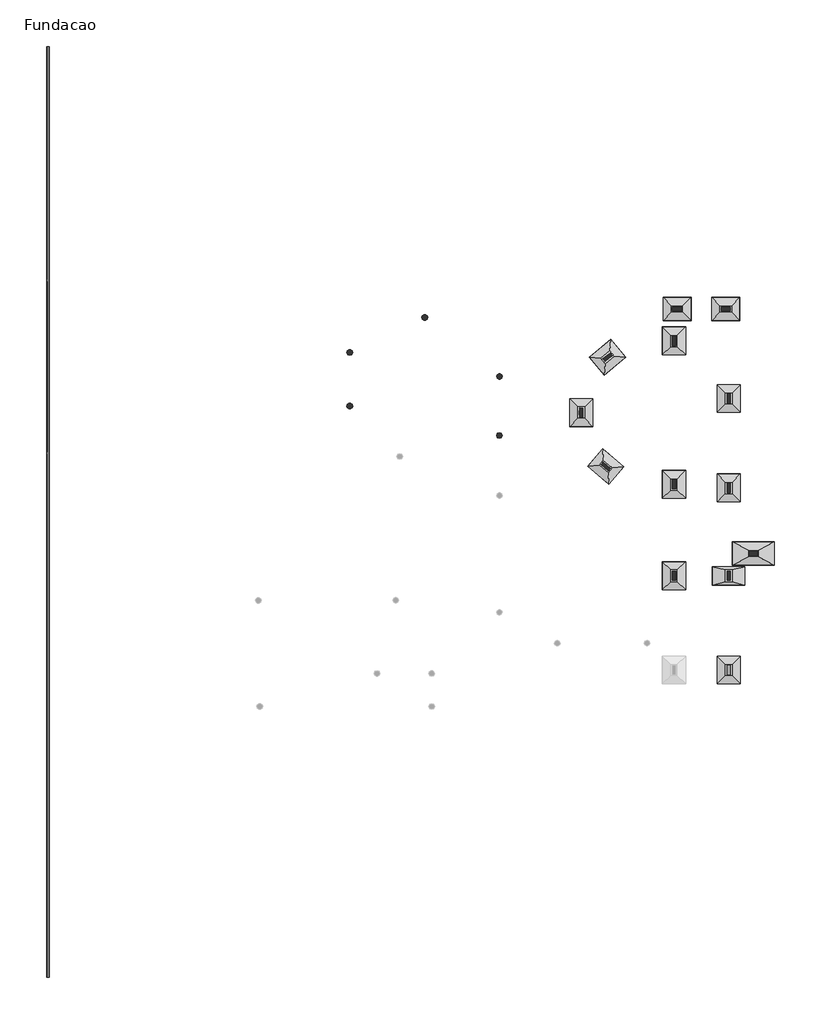
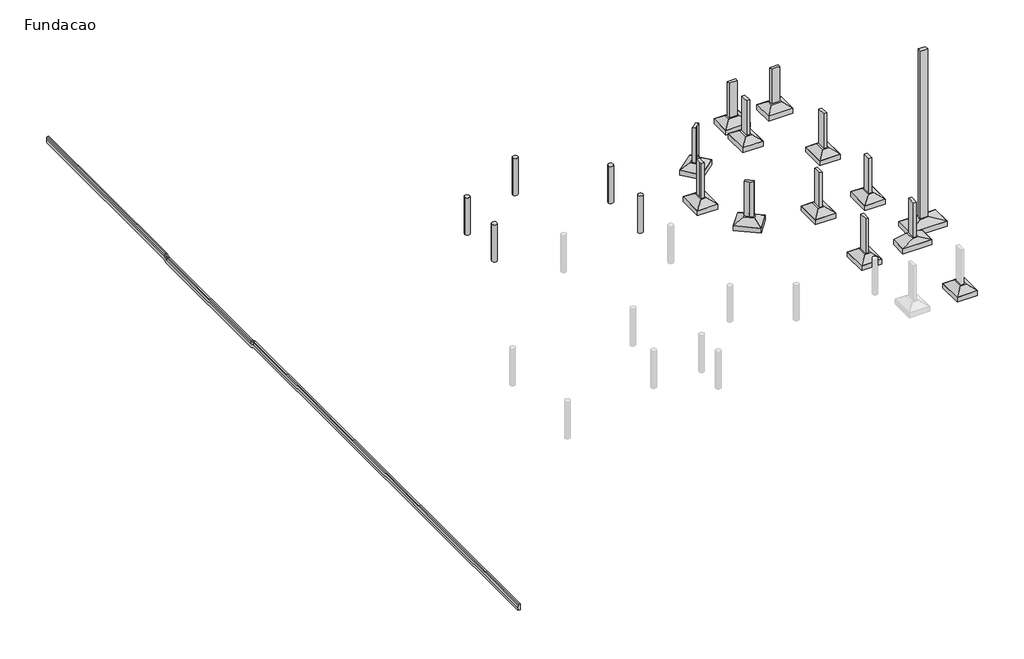
# One storey, part 2 of 2: 17 columns, 13 fasteners, 1 proxy.
"""IFC4 building model written with IfcOpenShell, lengths in millimetres."""

import ifcopenshell
import ifcopenshell.guid

model = None  # the IFC model being written
_history = None  # IfcOwnerHistory: only IFC2X3 demands one
_inside = {}  # id of a spatial element -> (the spatial element, [elements in it])
_under = {}  # id of a project, library or spatial element -> (it, [spatial elements below it])
_declared = {}  # id of a project -> (the project, [libraries it declares])
_typed = {}  # id of a type object -> (the type object, [elements of that type])
_made_of = {}  # id of a material, layer set ... -> (it, [elements and type objects made of it])


def new_model(schema):
    """Start an empty IFC model of exactly this schema.

    Asked for "IFC4X3", IfcOpenShell would pick the latest addendum, in which some entities
    have other attributes; the version numbers below select the first issue.
    IFC2X3 requires an IfcOwnerHistory on every rooted entity: one is made here for all.
    """
    global model, _history
    if schema == "IFC4X3":
        model = ifcopenshell.file(schema_version=(4, 3, 0, 0))
    else:
        model = ifcopenshell.file(schema=schema)
    _inside.clear()
    _under.clear()
    _declared.clear()
    _typed.clear()
    _made_of.clear()
    _history = None
    if model.schema == "IFC2X3":
        org = make("IfcOrganization", Name="unknown")
        user = make(
            "IfcPersonAndOrganization",
            ThePerson=make("IfcPerson", FamilyName="unknown"),
            TheOrganization=org,
        )
        app = make(
            "IfcApplication",
            ApplicationDeveloper=org,
            Version="unknown",
            ApplicationFullName="unknown",
            ApplicationIdentifier="unknown",
        )
        _history = make(
            "IfcOwnerHistory",
            OwningUser=user,
            OwningApplication=app,
            ChangeAction="ADDED",
            CreationDate=0,
        )
    return model


def make(cls, **values):
    """One entity of the class cls with the attributes given. An attribute that is None is left unset."""
    return model.create_entity(
        cls, **{name: value for name, value in values.items() if value is not None}
    )


def rooted(cls, **values):
    """An entity with a GlobalId (a new one), such as an element, a storey or a relation."""
    return make(cls, GlobalId=ifcopenshell.guid.new(), OwnerHistory=_history, **values)


def si_unit(unit_type, name, prefix=None):
    """IfcSIUnit, for example si_unit("LENGTHUNIT", "METRE", prefix="MILLI")."""
    return make("IfcSIUnit", UnitType=unit_type, Prefix=prefix, Name=name)


def assignment(units):
    """IfcUnitAssignment: the units of a project."""
    return None if units is None else make("IfcUnitAssignment", Units=units)


def point(xyz):
    """IfcCartesianPoint."""
    return None if xyz is None else make("IfcCartesianPoint", Coordinates=xyz)


def direction(xyz):
    """IfcDirection."""
    return None if xyz is None else make("IfcDirection", DirectionRatios=xyz)


def frame(location, z_axis=None, x_axis=None):
    """IfcAxis2Placement3D, a coordinate frame: its origin and axes. An axis left out is left unset."""
    return make(
        "IfcAxis2Placement3D",
        Location=point(location),
        Axis=direction(z_axis),
        RefDirection=direction(x_axis),
    )


def origin():
    """The frame at (0, 0, 0) with its axes left unset."""
    return frame((0.0, 0.0, 0.0))


def place(relative_to, where):
    """IfcLocalPlacement: puts the frame where relative to a parent placement (None: the world)."""
    return make(
        "IfcLocalPlacement", PlacementRelTo=relative_to, RelativePlacement=where
    )


def context(
    kind, dimensions, precision=None, world=None, true_north=None, identifier=None
):
    """IfcGeometricRepresentationContext, for example the 3D "Model" context."""
    return make(
        "IfcGeometricRepresentationContext",
        ContextIdentifier=identifier,
        ContextType=kind,
        CoordinateSpaceDimension=dimensions,
        Precision=precision,
        WorldCoordinateSystem=world,
        TrueNorth=true_north,
    )


def project(units=None, contexts=None):
    """IfcProject with its units and contexts."""
    return rooted(
        "IfcProject",
        Name="project",
        RepresentationContexts=contexts,
        UnitsInContext=assignment(units),
    )


def spatial(cls, under=None, at=None, **own):
    """A site, building, storey or space (cls), placed at a placement, below another one or the project."""
    s = rooted(cls, ObjectPlacement=at, **own)
    if under is not None:
        _under.setdefault(under.id(), (under, []))[1].append(s)
    return s


def polyline(points):
    """IfcPolyline through the points."""
    return make("IfcPolyline", Points=[point(p) for p in points])


def circle_curve(where, radius):
    """IfcCircle in the frame where."""
    return make("IfcCircle", Position=where, Radius=radius)


def ellipse_curve(where, semi_axis1, semi_axis2):
    """IfcEllipse in the frame where."""
    return make(
        "IfcEllipse", Position=where, SemiAxis1=semi_axis1, SemiAxis2=semi_axis2
    )


def outline(outer, holes=None, kind="AREA"):
    """IfcArbitraryClosedProfileDef: a profile drawn as a closed curve; with holes, ...WithVoids."""
    if holes is None:
        return make("IfcArbitraryClosedProfileDef", ProfileType=kind, OuterCurve=outer)
    return make(
        "IfcArbitraryProfileDefWithVoids",
        ProfileType=kind,
        OuterCurve=outer,
        InnerCurves=holes,
    )


def extrude(swept, where, along, depth):
    """IfcExtrudedAreaSolid: the profile swept, set in the frame where, extruded along a direction by depth."""
    return make(
        "IfcExtrudedAreaSolid",
        SweptArea=swept,
        Position=where,
        ExtrudedDirection=direction(along),
        Depth=depth,
    )


def faces_of(points, faces, orient=None, outer=None):
    """IfcFace entities. A face is a list of loops; a loop is a list of indices into points, from 0.

    orient and outer hold one flag for each loop. By default every Orientation is true, the
    first loop of a face is its IfcFaceOuterBound and the others are IfcFaceBound.
    """
    made = []
    for i, loops in enumerate(faces):
        bounds = []
        for j, loop in enumerate(loops):
            is_outer = j == 0 if outer is None else outer[i][j]
            bounds.append(
                make(
                    "IfcFaceOuterBound" if is_outer else "IfcFaceBound",
                    Bound=make("IfcPolyLoop", Polygon=[points[k] for k in loop]),
                    Orientation=True if orient is None else orient[i][j],
                )
            )
        made.append(make("IfcFace", Bounds=bounds))
    return made


def faceted_brep(points, faces, orient=None, outer=None, voids=None):
    """IfcFacetedBrep: a solid bounded by flat faces; with voids (closed shells), ...WithVoids."""
    shared = [point(p) for p in points]
    hull = make("IfcClosedShell", CfsFaces=faces_of(shared, faces, orient, outer))
    if voids is None:
        return make("IfcFacetedBrep", Outer=hull)
    return make(
        "IfcFacetedBrepWithVoids",
        Outer=hull,
        Voids=[
            make(cls, CfsFaces=faces_of(shared, fs, o, b)) for cls, fs, o, b in voids
        ],
    )


def shape(context_of_items, identifier, shape_type, items):
    """IfcShapeRepresentation: the items that make up one representation, for example the "Body"."""
    return make(
        "IfcShapeRepresentation",
        ContextOfItems=context_of_items,
        RepresentationIdentifier=identifier,
        RepresentationType=shape_type,
        Items=items,
    )


def source(mapping_origin, context_of_items, identifier, shape_type, items):
    """IfcRepresentationMap: a shape defined once, which mapped items show again and again."""
    return make(
        "IfcRepresentationMap",
        MappingOrigin=mapping_origin,
        MappedRepresentation=shape(context_of_items, identifier, shape_type, items),
    )


def transform(
    local_origin,
    x_axis=None,
    y_axis=None,
    z_axis=None,
    scale=None,
    scale2=None,
    scale3=None,
    uniform=True,
):
    """IfcCartesianTransformationOperator3D, or its non-uniform kind. x_axis, y_axis, z_axis: its Axis1, 2, 3."""
    if uniform:
        return make(
            "IfcCartesianTransformationOperator3D",
            Axis1=direction(x_axis),
            Axis2=direction(y_axis),
            LocalOrigin=point(local_origin),
            Scale=scale,
            Axis3=direction(z_axis),
        )
    return make(
        "IfcCartesianTransformationOperator3DnonUniform",
        Axis1=direction(x_axis),
        Axis2=direction(y_axis),
        LocalOrigin=point(local_origin),
        Scale=scale,
        Axis3=direction(z_axis),
        Scale2=scale2,
        Scale3=scale3,
    )


def mapped(mapping_source, mapping_target):
    """IfcMappedItem: shows the shape of a source again, moved by a transform."""
    return make(
        "IfcMappedItem", MappingSource=mapping_source, MappingTarget=mapping_target
    )


def made_of(thing, what):
    """Note that an element or type object is made of a material, layer set ...; save() writes the relation."""
    if what is not None:
        _made_of.setdefault(what.id(), (what, []))[1].append(thing)
    return thing


def element(
    cls,
    number,
    at=None,
    inside=None,
    cuts=None,
    type_object=None,
    material=None,
    context=None,
    identifier="Body",
    shape_type=None,
    held_by="IfcProductDefinitionShape",
    body=None,
    shapes=None,
    **own,
):
    """One element of the class cls, such as IfcWall. Its Tag is "e" and its number.

    at: its placement. inside: the storey or other place that contains it. cuts: it is an
    opening in that element (IfcRelVoidsElement). A single representation is given by context,
    identifier, shape_type and body (its items); several are given by shapes. held_by: the class
    of the entity that holds the representations. save() writes the other relations.
    """
    e = rooted(cls, Tag="e%d" % number, ObjectPlacement=at, **own)
    if body is not None:
        shapes = [shape(context, identifier, shape_type, body)]
    if shapes is not None:
        e.Representation = make(held_by, Representations=shapes)
    if inside is not None:
        _inside.setdefault(inside.id(), (inside, []))[1].append(e)
    if cuts is not None:
        rooted(
            "IfcRelVoidsElement", RelatingBuildingElement=cuts, RelatedOpeningElement=e
        )
    if type_object is not None:
        _typed.setdefault(type_object.id(), (type_object, []))[1].append(e)
    return made_of(e, material)


def aggregate(whole, parts):
    """IfcRelAggregates: a whole, such as a stair, and the parts it consists of."""
    return rooted("IfcRelAggregates", RelatingObject=whole, RelatedObjects=parts)


def save(model, path):
    """Write the relations noted so far, then the file.

    IfcRelAggregates (storeys below a building ...), IfcRelContainedInSpatialStructure (elements
    in a storey), IfcRelDefinesByType, IfcRelAssociatesMaterial and IfcRelDeclares: one each for
    every whole, place, type object, material and project.
    """
    for whole, parts in _under.values():
        aggregate(whole, parts)
    for where, things in _inside.values():
        rooted(
            "IfcRelContainedInSpatialStructure",
            RelatedElements=things,
            RelatingStructure=where,
        )
    for kind, things in _typed.values():
        rooted("IfcRelDefinesByType", RelatedObjects=things, RelatingType=kind)
    for what, things in _made_of.values():
        rooted("IfcRelAssociatesMaterial", RelatedObjects=things, RelatingMaterial=what)
    for by, libraries in _declared.values():
        rooted("IfcRelDeclares", RelatingContext=by, RelatedDefinitions=libraries)
    model.write(path)


def plane_surface(at):
    """IfcPlane: the flat surface through the origin of the frame at, square to its z axis."""
    return make("IfcPlane", Position=at)


def cylinder_surface(at, radius):
    """IfcCylindricalSurface: all points at the distance radius from the z axis of the frame at."""
    return make("IfcCylindricalSurface", Position=at, Radius=radius)


def advanced_brep(points, edges, surfaces, faces):
    """IfcAdvancedBrep: a solid bounded by faces that lie on surfaces and meet in shared edges.

    An edge is (start, end): straight between two places in points (the first is 0);
    or (start, end, curve); or (start, end, curve, False) where it runs against its curve.
    A face is (place in surfaces, loops), or (place, loops, False) where it looks against
    its surface's normal. A loop lists edges by number (the first is 1), with a minus sign
    where the edge is run from its end to its start. The first loop is the outer one.
    """
    corners = [point(p) for p in points]
    vertices = [make("IfcVertexPoint", VertexGeometry=c) for c in corners]
    made = []
    for start, end, *more in edges:
        made.append(
            make(
                "IfcEdgeCurve",
                EdgeStart=vertices[start],
                EdgeEnd=vertices[end],
                EdgeGeometry=more[0] if more else make("IfcPolyline", Points=[corners[start], corners[end]]),
                SameSense=more[1] if len(more) > 1 else True,
            )
        )
    hull = []
    for where, loops, *sense in faces:
        bounds = []
        for j, loop in enumerate(loops):
            ring = [make("IfcOrientedEdge", EdgeElement=made[abs(k) - 1], Orientation=k > 0) for k in loop]
            bounds.append(
                make(
                    "IfcFaceOuterBound" if j == 0 else "IfcFaceBound",
                    Bound=make("IfcEdgeLoop", EdgeList=ring),
                    Orientation=True,
                )
            )
        hull.append(make("IfcAdvancedFace", Bounds=bounds, FaceSurface=surfaces[where], SameSense=sense[0] if sense else True))
    return make("IfcAdvancedBrep", Outer=make("IfcClosedShell", CfsFaces=hull))


def meio_fio_meio_fio_c5939b1e(model_context):
    return source(origin(), model_context, "Body", "AdvancedBrep", [
        advanced_brep(
        [(-19460.281307, 17327.5225294, 100.0), (-19460.281307, 17327.5225294, -200.0), (-19580.281307, 17327.5225294, -200.0), (-19580.281307, 17327.5225294, -50.0), (-19560.334366, 17327.5225294, 74.7371665), (-19530.7107394, 17327.5225294, 100.0), (-19460.281307, 7304.4300153, 100.0), (-19460.281307, 7104.4300153, 20.0), (-19460.281307, 4.4300153, 20.0), (-19460.281307, -195.5699847, 100.0), (-19460.281307, -22700.938406, 100.0), (-19460.281307, -22700.938406, -200.0), (-19460.281307, -253.3447058, -200.0), (-19460.281307, -53.3447058, -280.0), (-19460.281307, 7162.2047364, -280.0), (-19460.281307, 7362.2047364, -200.0), (-19580.281307, 7362.2047364, -200.0), (-19580.281307, 7162.2047364, -280.0), (-19580.281307, -53.3447058, -280.0), (-19580.281307, -253.3447058, -200.0), (-19580.281307, -22700.938406, -200.0), (-19580.281307, -22700.938406, -50.0), (-19580.281307, -224.4573452, -50.0), (-19580.281307, -24.4573452, -130.0), (-19580.281307, 7133.3173758, -130.0), (-19580.281307, 7333.3173758, -50.0), (-19560.334366, 7309.2951925, 74.7371665), (-19530.7107394, 7304.4300153, 100.0), (-19560.334366, 7109.2951925, -5.2628335), (-19530.7107394, 7104.4300153, 20.0), (-19560.334366, -0.4351619, -5.2628335), (-19530.7107394, 4.4300153, 20.0), (-19560.334366, -200.4351619, 74.7371665), (-19530.7107394, -195.5699847, 100.0), (-19530.7107394, -22700.938406, 100.0), (-19560.334366, -22700.938406, 74.7371665)],
        [
            (0, 1),
            (1, 2),
            (2, 3),
            (3, 4),
            (4, 5, circle_curve(frame((-19530.7107394, 17327.5225294, 70.0), z_axis=(0.0, 1.0, 0.0), x_axis=(-1.0, 0.0, 0.0)), 30.0)),
            (5, 0),
            (0, 6),
            (6, 7),
            (7, 8),
            (8, 9),
            (9, 10),
            (10, 11),
            (11, 12),
            (12, 13),
            (13, 14),
            (14, 15),
            (15, 1),
            (15, 16),
            (16, 2),
            (16, 17),
            (17, 18),
            (18, 19),
            (19, 20),
            (20, 21),
            (21, 22),
            (22, 23),
            (23, 24),
            (24, 25),
            (25, 3),
            (25, 26),
            (26, 4),
            (26, 27, ellipse_curve(frame((-19530.7107394, 7310.2074874, 70.0), z_axis=(0.0, 0.9819563867314226, 0.18910752115494767), x_axis=(0.0, 0.18910752115494667, -0.9819563867314226)), 30.551255, 30.0)),
            (27, 5),
            (27, 6),
            (14, 17),
            (24, 28),
            (28, 26),
            (28, 29, ellipse_curve(frame((-19530.7107394, 7110.2074874, -10.0), z_axis=(0.0, 0.9819563867314226, 0.18910752115494764), x_axis=(0.0, -0.18910752115494842, 0.9819563867314223)), 30.551255, 30.0)),
            (29, 27),
            (29, 7),
            (13, 18),
            (23, 30),
            (30, 28),
            (30, 31, ellipse_curve(frame((-19530.7107394, -1.3474568, -10.0), z_axis=(0.0, 0.9819563867314217, -0.1891075211549513), x_axis=(0.0, 0.18910752115495252, 0.9819563867314217)), 30.551255, 30.0)),
            (31, 29),
            (31, 8),
            (12, 19),
            (22, 32),
            (32, 30),
            (32, 33, ellipse_curve(frame((-19530.7107394, -201.3474568, 70.0), z_axis=(0.0, 0.9819563867314217, -0.18910752115495139), x_axis=(0.0, -0.18910752115495078, -0.9819563867314218)), 30.551255, 30.0)),
            (33, 31),
            (33, 9),
            (10, 34),
            (34, 35, circle_curve(frame((-19530.7107394, -22700.938406, 70.0), z_axis=(0.0, -1.0, 0.0), x_axis=(-1.0, 0.0, 0.0)), 30.0)),
            (35, 21),
            (20, 11),
            (35, 32),
            (34, 33),
        ],
        [
            plane_surface(frame((-19460.281307, 17327.5225294, 100.0), z_axis=(0.0, 1.0, 0.0), x_axis=(0.0, 0.0, 1.0))),
            plane_surface(frame((-19460.281307, 17327.5225294, 100.0), z_axis=(1.0, 0.0, 0.0), x_axis=(0.0, -1.0, 0.0))),
            plane_surface(frame((-19460.281307, 17327.5225294, -200.0), z_axis=(0.0, 0.0, -1.0), x_axis=(0.0, -1.0, 0.0))),
            plane_surface(frame((-19580.281307, 17327.5225294, -200.0), z_axis=(-1.0, 0.0, 0.0), x_axis=(0.0, -1.0, 0.0))),
            plane_surface(frame((-19580.281307, 17327.5225294, -50.0), z_axis=(-0.9874542202157147, 0.0, 0.15790555081495689), x_axis=(0.0, -1.0, 0.0))),
            cylinder_surface(frame((-19530.7107394, 17327.5225294, 70.0), z_axis=(0.0, 1.0, 0.0), x_axis=(-1.0, 0.0, 0.0)), 30.0),
            plane_surface(frame((-19530.7107394, 17327.5225294, 100.0), z_axis=(0.0, 0.0, 1.0), x_axis=(0.0, -1.0, 0.0))),
            plane_surface(frame((-19460.281307, 7362.2047364, -200.0), z_axis=(0.0, 0.3713906763540969, -0.9284766908852621), x_axis=(0.0, -0.9284766908852621, -0.3713906763540969))),
            plane_surface(frame((-19580.281307, 7333.3173758, -50.0), z_axis=(-0.9874542202157147, -0.05864464931723302, 0.1466116232930858), x_axis=(0.0, -0.9284766908852622, -0.3713906763540966))),
            cylinder_surface(frame((-19530.7107394, 7315.5717356, 72.1456993), z_axis=(0.0, 0.9284766908852621, 0.3713906763540969), x_axis=(-1.0, 0.0, 0.0)), 30.0),
            plane_surface(frame((-19530.7107394, 7304.4300153, 100.0), z_axis=(0.0, -0.37139067635409667, 0.9284766908852622), x_axis=(0.0, -0.9284766908852622, -0.37139067635409667))),
            plane_surface(frame((-19460.281307, 7162.2047364, -280.0), z_axis=(0.0, 0.0, -1.0), x_axis=(0.0, -1.0, 0.0))),
            plane_surface(frame((-19580.281307, 7133.3173758, -130.0), z_axis=(-0.9874542202157146, 0.0, 0.15790555081495686), x_axis=(0.0, -1.0, 0.0))),
            cylinder_surface(frame((-19530.7107394, 7104.4300153, -10.0), z_axis=(0.0, 1.0, 0.0), x_axis=(-1.0, 0.0, 0.0)), 30.0),
            plane_surface(frame((-19530.7107394, 7104.4300153, 20.0), z_axis=(0.0, 0.0, 1.0), x_axis=(0.0, -1.0, 0.0))),
            plane_surface(frame((-19460.281307, -53.3447058, -280.0), z_axis=(0.0, -0.37139067635410367, -0.9284766908852594), x_axis=(0.0, -0.9284766908852594, 0.37139067635410367))),
            plane_surface(frame((-19580.281307, -24.4573452, -130.0), z_axis=(-0.9874542202157147, 0.05864464931723411, 0.14661162329308536), x_axis=(0.0, -0.9284766908852594, 0.37139067635410355))),
            cylinder_surface(frame((-19530.7107394, -6.711705, -7.8543007), z_axis=(0.0, 0.9284766908852593, -0.3713906763541038), x_axis=(-1.0, 0.0, 0.0)), 30.0),
            plane_surface(frame((-19530.7107394, 4.4300153, 20.0), z_axis=(0.0, 0.3713906763541038, 0.9284766908852593), x_axis=(0.0, -0.9284766908852593, 0.3713906763541038))),
            plane_surface(frame((-19460.281307, -22700.938406, 100.0), z_axis=(0.0, -1.0, 0.0), x_axis=(0.0, 0.0, 1.0))),
            plane_surface(frame((-19460.281307, -253.3447058, -200.0), z_axis=(0.0, 0.0, -1.0), x_axis=(0.0, -1.0, 0.0))),
            plane_surface(frame((-19580.281307, -224.4573452, -50.0), z_axis=(-0.9874542202157146, 0.0, 0.15790555081495683), x_axis=(0.0, -1.0, 0.0))),
            cylinder_surface(frame((-19530.7107394, -195.5699847, 70.0), z_axis=(0.0, 1.0, 0.0), x_axis=(-1.0, 0.0, 0.0)), 30.0),
            plane_surface(frame((-19530.7107394, -195.5699847, 100.0), z_axis=(0.0, 0.0, 1.0), x_axis=(0.0, -1.0, 0.0))),
        ],
        [
            (0, [[1, 2, 3, 4, 5, 6]]),
            (1, [[-1, 7, 8, 9, 10, 11, 12, 13, 14, 15, 16, 17]]),
            (2, [[-2, -17, 18, 19]]),
            (3, [[-3, -19, 20, 21, 22, 23, 24, 25, 26, 27, 28, 29]]),
            (4, [[-4, -29, 30, 31]]),
            (5, [[-5, -31, 32, 33]]),
            (6, [[-6, -33, 34, -7]]),
            (7, [[-18, -16, 35, -20]]),
            (8, [[-30, -28, 36, 37]]),
            (9, [[-32, -37, 38, 39]]),
            (10, [[-34, -39, 40, -8]]),
            (11, [[-35, -15, 41, -21]]),
            (12, [[-36, -27, 42, 43]]),
            (13, [[-38, -43, 44, 45]]),
            (14, [[-40, -45, 46, -9]]),
            (15, [[-41, -14, 47, -22]]),
            (16, [[-42, -26, 48, 49]]),
            (17, [[-44, -49, 50, 51]]),
            (18, [[-46, -51, 52, -10]]),
            (19, [[53, 54, 55, -24, 56, -12]]),
            (20, [[-47, -13, -56, -23]]),
            (21, [[-48, -25, -55, 57]]),
            (22, [[-50, -57, -54, 58]]),
            (23, [[-52, -58, -53, -11]]),
        ],
    ),
    ])


def s14_8166d2be(model_context):
    return source(origin(), model_context, "Body", "SolidModel", [
        faceted_brep([(-55.0, 0.0, 0.0), (-345.0, 0.0, 0.0), (-345.0, -400.0, 0.0), (-55.0, -400.0, 0.0), (300.0, 700.0, -250.0), (300.0, -1100.0, -250.0), (-700.0, -1100.0, -250.0), (-700.0, 700.0, -250.0)], [[[0, 1, 2, 3]], [[4, 5, 6, 7]], [[4, 7, 1, 0]], [[7, 6, 2, 1]], [[6, 5, 3, 2]], [[5, 4, 0, 3]]]),
        extrude(outline(polyline([(300.0, 700.0), (300.0, -1100.0), (-700.0, -1100.0), (-700.0, 700.0), (300.0, 700.0)])), frame((0.0, 0.0, -500.0), z_axis=(0.0, 0.0, 1.0), x_axis=(1.0, 0.0, 0.0)), (0.0, 0.0, 1.0), 250.0),
    ])


def sps1_6b3be553(model_context):
    return source(origin(), model_context, "Body", "SolidModel", [
        faceted_brep([(-55.0, 50.0, 0.0), (-345.0, 50.0, 0.0), (-345.0, -450.0, 0.0), (-55.0, -450.0, 0.0), (300.0, 400.0, -250.0), (300.0, -800.0, -250.0), (-700.0, -800.0, -250.0), (-700.0, 400.0, -250.0)], [[[0, 1, 2, 3]], [[4, 5, 6, 7]], [[4, 7, 1, 0]], [[7, 6, 2, 1]], [[6, 5, 3, 2]], [[5, 4, 0, 3]]]),
        extrude(outline(polyline([(300.0, 400.0), (300.0, -800.0), (-700.0, -800.0), (-700.0, 400.0), (300.0, 400.0)])), frame((0.0, 0.0, -500.0), z_axis=(0.0, 0.0, 1.0), x_axis=(1.0, 0.0, 0.0)), (0.0, 0.0, 1.0), 250.0),
    ])


def sps11_3ae28187(model_context):
    return source(origin(), model_context, "Body", "SolidModel", [
        faceted_brep([(-55.0, 50.0, 0.0), (-345.0, 50.0, 0.0), (-345.0, -450.0, 0.0), (-55.0, -450.0, 0.0), (500.0, 200.0, -250.0), (500.0, -600.0, -250.0), (-900.0, -600.0, -250.0), (-900.0, 200.0, -250.0)], [[[0, 1, 2, 3]], [[4, 5, 6, 7]], [[4, 7, 1, 0]], [[7, 6, 2, 1]], [[6, 5, 3, 2]], [[5, 4, 0, 3]]]),
        extrude(outline(polyline([(500.0, 200.0), (500.0, -600.0), (-900.0, -600.0), (-900.0, 200.0), (500.0, 200.0)])), frame((0.0, 0.0, -500.0), z_axis=(0.0, 0.0, 1.0), x_axis=(1.0, 0.0, 0.0)), (0.0, 0.0, 1.0), 250.0),
    ])


model = new_model("IFC4")

# Units and contexts
model_context = context("Model", 3, world=origin())
ifc_project = project(units=[si_unit("LENGTHUNIT", "METRE", prefix="MILLI")], contexts=[model_context])

# Site, building, storey
site = spatial("IfcSite", under=ifc_project)
building = spatial("IfcBuilding", under=site)
storey = spatial("IfcBuildingStorey", under=building, Name="Fundacao", Elevation=-1200.0)

# Proxy
placement = place(None, origin())
meio_fio_meio_fio_shape = meio_fio_meio_fio_c5939b1e(model_context)
element("IfcBuildingElementProxy", 1, Name="MEIO-FIO : MEIO-FIO", ObjectType="MEIO-FIO : MEIO-FIO", at=placement, inside=storey, context=model_context, shape_type="MappedRepresentation", body=[
    mapped(meio_fio_meio_fio_shape, transform((0.0, 0.0, 0.0), x_axis=(1.0, 0.0, 0.0), y_axis=(0.0, 1.0, 0.0), z_axis=(0.0, 0.0, 1.0))),
])

# Columns
element("IfcColumn", 2, ObjectType="TQS - Pilar circular : TQS - Pilar circular 25.0cm", at=placement, inside=storey, context=model_context, shape_type="AdvancedBrep", body=[
    advanced_brep(
    [(-3446.281307, 5679.4300153, -1500.0), (-3196.281307, 5679.4300153, -1500.0), (-3446.281307, 5679.4300153, 430.0), (-3402.499945, 5774.4486073, 430.0), (-3240.0409229, 5774.4300153, 430.0), (-3196.281307, 5679.4300153, 430.0), (-3240.0409229, 5584.4300153, 430.0), (-3402.499945, 5584.4114233, 430.0)],
    [
        (0, 1, circle_curve(frame((-3321.281307, 5679.4300153, -1500.0), z_axis=(0.0, 0.0, -1.0), x_axis=(1.0, 0.0, 0.0)), 125.0)),
        (1, 0, circle_curve(frame((-3321.281307, 5679.4300153, -1500.0), z_axis=(0.0, 0.0, -1.0), x_axis=(1.0, 0.0, 0.0)), 125.0)),
        (2, 3, circle_curve(frame((-3321.281307, 5679.4300153, 430.0), z_axis=(0.0, 0.0, -1.0), x_axis=(1.0, 0.0, 0.0)), 125.0)),
        (3, 4, circle_curve(frame((-3321.281307, 5679.4300153, 430.0), z_axis=(0.0, 0.0, -1.0), x_axis=(1.0, 0.0, 0.0)), 125.0)),
        (4, 5, circle_curve(frame((-3321.281307, 5679.4300153, 430.0), z_axis=(0.0, 0.0, -1.0), x_axis=(1.0, 0.0, 0.0)), 125.0)),
        (5, 1),
        (0, 2),
        (5, 6, circle_curve(frame((-3321.281307, 5679.4300153, 430.0), z_axis=(0.0, 0.0, -1.0), x_axis=(1.0, 0.0, 0.0)), 125.0)),
        (6, 7, circle_curve(frame((-3321.281307, 5679.4300153, 430.0), z_axis=(0.0, 0.0, -1.0), x_axis=(1.0, 0.0, 0.0)), 125.0)),
        (7, 2, circle_curve(frame((-3321.281307, 5679.4300153, 430.0), z_axis=(0.0, 0.0, -1.0), x_axis=(1.0, 0.0, 0.0)), 125.0)),
    ],
    [
        plane_surface(frame((-3196.281307, 5679.4300153, -1500.0), z_axis=(0.0, 0.0, -1.0), x_axis=(0.0, -1.0, 0.0))),
        cylinder_surface(frame((-3321.281307, 5679.4300153, -1500.0), z_axis=(0.0, 0.0, 1.0), x_axis=(1.0, 0.0, 0.0)), 125.0),
        plane_surface(frame((-3196.281307, 5679.4300153, 430.0), z_axis=(0.0, 0.0, 1.0), x_axis=(0.0, 1.0, 0.0))),
    ],
    [
        (0, [[1, 2]]),
        (1, [[3, 4, 5, 6, -1, 7]]),
        (1, [[8, 9, 10, -7, -2, -6]]),
        (2, [[-10, -9, -8, -5, -4, -3]]),
    ],
),
])
element("IfcColumn", 3, ObjectType="TQS - Pilar circular : TQS - Pilar circular 25.0cm", at=placement, inside=storey, context=model_context, shape_type="AdvancedBrep", body=[
    advanced_brep(
    [(-232.281307, 604.4300152, -1500.0), (17.718693, 604.4300152, -1500.0), (-232.281307, 604.4300152, 430.0), (-202.281307, 685.6703993, 430.0), (-12.281307, 685.6703993, 430.0), (17.718693, 604.4300152, 430.0), (-12.281307, 523.1896312, 430.0), (-202.281307, 523.1896312, 430.0)],
    [
        (0, 1, circle_curve(frame((-107.281307, 604.4300152, -1500.0), z_axis=(0.0, 0.0, -1.0), x_axis=(1.0, 0.0, 0.0)), 125.0)),
        (1, 0, circle_curve(frame((-107.281307, 604.4300152, -1500.0), z_axis=(0.0, 0.0, -1.0), x_axis=(1.0, 0.0, 0.0)), 125.0)),
        (2, 3, circle_curve(frame((-107.281307, 604.4300152, 430.0), z_axis=(0.0, 0.0, -1.0), x_axis=(1.0, 0.0, 0.0)), 125.0)),
        (3, 4, circle_curve(frame((-107.281307, 604.4300152, 430.0), z_axis=(0.0, 0.0, -1.0), x_axis=(1.0, 0.0, 0.0)), 125.0)),
        (4, 5, circle_curve(frame((-107.281307, 604.4300152, 430.0), z_axis=(0.0, 0.0, -1.0), x_axis=(1.0, 0.0, 0.0)), 125.0)),
        (5, 1),
        (0, 2),
        (5, 6, circle_curve(frame((-107.281307, 604.4300152, 430.0), z_axis=(0.0, 0.0, -1.0), x_axis=(1.0, 0.0, 0.0)), 125.0)),
        (6, 7, circle_curve(frame((-107.281307, 604.4300152, 430.0), z_axis=(0.0, 0.0, -1.0), x_axis=(1.0, 0.0, 0.0)), 125.0)),
        (7, 2, circle_curve(frame((-107.281307, 604.4300152, 430.0), z_axis=(0.0, 0.0, -1.0), x_axis=(1.0, 0.0, 0.0)), 125.0)),
    ],
    [
        plane_surface(frame((17.718693, 604.4300152, -1500.0), z_axis=(0.0, 0.0, -1.0), x_axis=(0.0, -1.0, 0.0))),
        cylinder_surface(frame((-107.281307, 604.4300152, -1500.0), z_axis=(0.0, 0.0, 1.0), x_axis=(1.0, 0.0, 0.0)), 125.0),
        plane_surface(frame((17.718693, 604.4300152, 430.0), z_axis=(0.0, 0.0, 1.0), x_axis=(0.0, 1.0, 0.0))),
    ],
    [
        (0, [[1, 2]]),
        (1, [[3, 4, 5, 6, -1, 7]]),
        (1, [[8, 9, 10, -7, -2, -6]]),
        (2, [[-10, -9, -8, -5, -4, -3]]),
    ],
),
])
element("IfcColumn", 4, ObjectType="TQS - Pilar circular : TQS - Pilar circular 25.0cm", at=placement, inside=storey, context=model_context, shape_type="AdvancedBrep", body=[
    advanced_brep(
    [(-232.281307, 3141.9300152, -1500.0), (17.718693, 3141.9300152, -1500.0), (-232.281307, 3141.9300152, 430.0), (-202.281307, 3223.1703993, 430.0), (-12.281307, 3223.1703993, 430.0), (17.718693, 3141.9300152, 430.0), (-12.281307, 3060.6896312, 430.0), (-202.281307, 3060.6896312, 430.0)],
    [
        (0, 1, circle_curve(frame((-107.281307, 3141.9300152, -1500.0), z_axis=(0.0, 0.0, -1.0), x_axis=(1.0, 0.0, 0.0)), 125.0)),
        (1, 0, circle_curve(frame((-107.281307, 3141.9300152, -1500.0), z_axis=(0.0, 0.0, -1.0), x_axis=(1.0, 0.0, 0.0)), 125.0)),
        (2, 3, circle_curve(frame((-107.281307, 3141.9300152, 430.0), z_axis=(0.0, 0.0, -1.0), x_axis=(1.0, 0.0, 0.0)), 125.0)),
        (3, 4, circle_curve(frame((-107.281307, 3141.9300152, 430.0), z_axis=(0.0, 0.0, -1.0), x_axis=(1.0, 0.0, 0.0)), 125.0)),
        (4, 5, circle_curve(frame((-107.281307, 3141.9300152, 430.0), z_axis=(0.0, 0.0, -1.0), x_axis=(1.0, 0.0, 0.0)), 125.0)),
        (5, 1),
        (0, 2),
        (5, 6, circle_curve(frame((-107.281307, 3141.9300152, 430.0), z_axis=(0.0, 0.0, -1.0), x_axis=(1.0, 0.0, 0.0)), 125.0)),
        (6, 7, circle_curve(frame((-107.281307, 3141.9300152, 430.0), z_axis=(0.0, 0.0, -1.0), x_axis=(1.0, 0.0, 0.0)), 125.0)),
        (7, 2, circle_curve(frame((-107.281307, 3141.9300152, 430.0), z_axis=(0.0, 0.0, -1.0), x_axis=(1.0, 0.0, 0.0)), 125.0)),
    ],
    [
        plane_surface(frame((17.718693, 3141.9300152, -1500.0), z_axis=(0.0, 0.0, -1.0), x_axis=(0.0, -1.0, 0.0))),
        cylinder_surface(frame((-107.281307, 3141.9300152, -1500.0), z_axis=(0.0, 0.0, 1.0), x_axis=(1.0, 0.0, 0.0)), 125.0),
        plane_surface(frame((17.718693, 3141.9300152, 430.0), z_axis=(0.0, 0.0, 1.0), x_axis=(0.0, 1.0, 0.0))),
    ],
    [
        (0, [[1, 2]]),
        (1, [[3, 4, 5, 6, -1, 7]]),
        (1, [[8, 9, 10, -7, -2, -6]]),
        (2, [[-10, -9, -8, -5, -4, -3]]),
    ],
),
])
element("IfcColumn", 5, ObjectType="TQS - Pilar circular : TQS - Pilar circular 25.0cm", at=placement, inside=storey, context=model_context, shape_type="AdvancedBrep", body=[
    advanced_brep(
    [(-6671.281307, 4171.2050153, -1500.0), (-6421.281307, 4171.2050153, -1500.0), (-6671.281307, 4171.2050153, 430.0), (-6630.281307, 4263.7739086, 430.0), (-6440.281307, 4237.4545436, 430.0), (-6421.281307, 4171.2050153, 430.0), (-6440.281307, 4104.955487, 430.0), (-6630.281307, 4078.636122, 430.0)],
    [
        (0, 1, circle_curve(frame((-6546.281307, 4171.2050153, -1500.0), z_axis=(0.0, 0.0, -1.0), x_axis=(1.0, 0.0, 0.0)), 125.0)),
        (1, 0, circle_curve(frame((-6546.281307, 4171.2050153, -1500.0), z_axis=(0.0, 0.0, -1.0), x_axis=(1.0, 0.0, 0.0)), 125.0)),
        (2, 3, circle_curve(frame((-6546.281307, 4171.2050153, 430.0), z_axis=(0.0, 0.0, -1.0), x_axis=(1.0, 0.0, 0.0)), 125.0)),
        (3, 4, circle_curve(frame((-6546.281307, 4171.2050153, 430.0), z_axis=(0.0, 0.0, -1.0), x_axis=(1.0, 0.0, 0.0)), 125.0)),
        (4, 5, circle_curve(frame((-6546.281307, 4171.2050153, 430.0), z_axis=(0.0, 0.0, -1.0), x_axis=(1.0, 0.0, 0.0)), 125.0)),
        (5, 1),
        (0, 2),
        (5, 6, circle_curve(frame((-6546.281307, 4171.2050153, 430.0), z_axis=(0.0, 0.0, -1.0), x_axis=(1.0, 0.0, 0.0)), 125.0)),
        (6, 7, circle_curve(frame((-6546.281307, 4171.2050153, 430.0), z_axis=(0.0, 0.0, -1.0), x_axis=(1.0, 0.0, 0.0)), 125.0)),
        (7, 2, circle_curve(frame((-6546.281307, 4171.2050153, 430.0), z_axis=(0.0, 0.0, -1.0), x_axis=(1.0, 0.0, 0.0)), 125.0)),
    ],
    [
        plane_surface(frame((-6421.281307, 4171.2050153, -1500.0), z_axis=(0.0, 0.0, -1.0), x_axis=(0.0, -1.0, 0.0))),
        cylinder_surface(frame((-6546.281307, 4171.2050153, -1500.0), z_axis=(0.0, 0.0, 1.0), x_axis=(1.0, 0.0, 0.0)), 125.0),
        plane_surface(frame((-6421.281307, 4171.2050153, 430.0), z_axis=(0.0, 0.0, 1.0), x_axis=(0.0, 1.0, 0.0))),
    ],
    [
        (0, [[1, 2]]),
        (1, [[3, 4, 5, 6, -1, 7]]),
        (1, [[8, 9, 10, -7, -2, -6]]),
        (2, [[-10, -9, -8, -5, -4, -3]]),
    ],
),
])
element("IfcColumn", 6, ObjectType="TQS - Pilar circular : TQS - Pilar circular 25.0cm", at=placement, inside=storey, context=model_context, shape_type="AdvancedBrep", body=[
    advanced_brep(
    [(-6666.2813069, 1866.7050153, -1500.0), (-6416.2813069, 1866.7050153, -1500.0), (-6666.2813069, 1866.7050153, 430.0), (-6630.281307, 1954.4774483, 430.0), (-6440.281307, 1940.3528259, 430.0), (-6416.2813069, 1866.7050153, 430.0), (-6440.281307, 1793.0572047, 430.0), (-6630.281307, 1778.9325823, 430.0)],
    [
        (0, 1, circle_curve(frame((-6541.2813069, 1866.7050153, -1500.0), z_axis=(0.0, 0.0, -1.0), x_axis=(1.0, 0.0, 0.0)), 125.0)),
        (1, 0, circle_curve(frame((-6541.2813069, 1866.7050153, -1500.0), z_axis=(0.0, 0.0, -1.0), x_axis=(1.0, 0.0, 0.0)), 125.0)),
        (2, 3, circle_curve(frame((-6541.2813069, 1866.7050153, 430.0), z_axis=(0.0, 0.0, -1.0), x_axis=(1.0, 0.0, 0.0)), 125.0)),
        (3, 4, circle_curve(frame((-6541.2813069, 1866.7050153, 430.0), z_axis=(0.0, 0.0, -1.0), x_axis=(1.0, 0.0, 0.0)), 125.0)),
        (4, 5, circle_curve(frame((-6541.2813069, 1866.7050153, 430.0), z_axis=(0.0, 0.0, -1.0), x_axis=(1.0, 0.0, 0.0)), 125.0)),
        (5, 1),
        (0, 2),
        (5, 6, circle_curve(frame((-6541.2813069, 1866.7050153, 430.0), z_axis=(0.0, 0.0, -1.0), x_axis=(1.0, 0.0, 0.0)), 125.0)),
        (6, 7, circle_curve(frame((-6541.2813069, 1866.7050153, 430.0), z_axis=(0.0, 0.0, -1.0), x_axis=(1.0, 0.0, 0.0)), 125.0)),
        (7, 2, circle_curve(frame((-6541.2813069, 1866.7050153, 430.0), z_axis=(0.0, 0.0, -1.0), x_axis=(1.0, 0.0, 0.0)), 125.0)),
    ],
    [
        plane_surface(frame((-6416.2813069, 1866.7050153, -1500.0), z_axis=(0.0, 0.0, -1.0), x_axis=(0.0, -1.0, 0.0))),
        cylinder_surface(frame((-6541.2813069, 1866.7050153, -1500.0), z_axis=(0.0, 0.0, 1.0), x_axis=(1.0, 0.0, 0.0)), 125.0),
        plane_surface(frame((-6416.2813069, 1866.7050153, 430.0), z_axis=(0.0, 0.0, 1.0), x_axis=(0.0, 1.0, 0.0))),
    ],
    [
        (0, [[1, 2]]),
        (1, [[3, 4, 5, 6, -1, 7]]),
        (1, [[8, 9, 10, -7, -2, -6]]),
        (2, [[-10, -9, -8, -5, -4, -3]]),
    ],
),
])
element("IfcColumn", 7, ObjectType="TQS - Pilar retangular : 14.0 x 40.0", at=placement, inside=storey, context=model_context, shape_type="Brep", body=[
    faceted_brep([(9822.718693, 5969.4300153, -1450.0), (9682.718693, 5969.4300153, -1450.0), (9422.718693, 5969.4300153, -1450.0), (9422.718693, 6109.4300153, -1450.0), (9822.718693, 6109.4300153, -1450.0), (9822.718693, 5969.4300153, 350.0), (9682.718693, 5969.4300153, 350.0), (9422.718693, 5969.4300153, 350.0), (9422.718693, 6109.4300153, 350.0), (9822.718693, 6109.4300153, 350.0)], [[[0, 1, 2, 3, 4]], [[5, 6, 7, 2, 1, 0]], [[7, 8, 3, 2]], [[8, 9, 4, 3]], [[9, 5, 0, 4]], [[5, 9, 8, 7, 6]]]),
])
element("IfcColumn", 8, ObjectType="TQS - Pilar retangular : 14.0 x 40.0", at=placement, inside=storey, context=model_context, shape_type="Brep", body=[
    faceted_brep([(7734.718693, 5969.4300153, -1450.0), (7474.7218272, 5969.4300153, -1450.0), (7334.718693, 5969.4300153, -1450.0), (7334.718693, 6109.4300153, -1450.0), (7734.718693, 6109.4300153, -1450.0), (7734.718693, 5969.4300153, 350.0), (7474.7218272, 5969.4300153, 350.0), (7334.718693, 5969.4300153, 350.0), (7334.718693, 6109.4300153, 350.0), (7734.718693, 6109.4300153, 350.0)], [[[0, 1, 2, 3, 4]], [[5, 6, 7, 2, 1, 0]], [[7, 8, 3, 2]], [[8, 9, 4, 3]], [[9, 5, 0, 4]], [[5, 9, 8, 7, 6]]]),
])
element("IfcColumn", 9, ObjectType="TQS - Pilar retangular : 14.0 x 40.0", at=placement, inside=storey, context=model_context, shape_type="Brep", body=[
    faceted_brep([(7334.7218272, 4470.7003679, -1450.0), (7334.7218272, 4614.8968948, -1450.0), (7334.7218272, 4870.7003679, -1450.0), (7474.7218272, 4870.7003679, -1450.0), (7474.7218272, 4470.7003679, -1450.0), (7334.7218272, 4470.7003679, -1250.0), (7334.7218272, 4470.7003679, 350.0), (7334.7218272, 4614.8968948, 350.0), (7334.7218272, 4870.7003679, 350.0), (7474.7218272, 4870.7003679, 350.0), (7474.7218272, 4870.7003679, -1250.0), (7474.7218272, 4470.7003679, 350.0), (7474.7218272, 4470.7003679, -1250.0)], [[[0, 1, 2, 3, 4]], [[2, 1, 0, 5, 6, 7, 8]], [[3, 2, 8, 9, 10]], [[4, 3, 10, 9, 11, 12]], [[0, 4, 12, 11, 6, 5]], [[8, 7, 6, 11, 9]]]),
])
element("IfcColumn", 10, ObjectType="TQS - Pilar retangular : 14.0 x 40.0", at=placement, inside=storey, context=model_context, shape_type="Brep", body=[
    faceted_brep([(7334.718693, -1696.0936198, -1450.0), (7334.718693, -1440.2725066, -1450.0), (7334.718693, -1296.0936198, -1450.0), (7474.718693, -1296.0936198, -1450.0), (7474.718693, -1696.0936198, -1450.0), (7334.718693, -1696.0936198, 350.0), (7334.718693, -1440.2725066, 350.0), (7334.718693, -1296.0936198, 350.0), (7334.718693, -1296.0936198, -1250.0), (7474.718693, -1296.0936198, 350.0), (7474.718693, -1296.0936198, -1250.0), (7474.718693, -1696.0936198, 350.0), (7474.718693, -1696.0936198, -1250.0)], [[[0, 1, 2, 3, 4]], [[2, 1, 0, 5, 6, 7, 8]], [[3, 2, 8, 7, 9, 10]], [[4, 3, 10, 9, 11, 12]], [[0, 4, 12, 11, 5]], [[7, 6, 5, 11, 9]]]),
])
element("IfcColumn", 11, ObjectType="TQS - Pilar retangular : 14.0 x 40.0", at=placement, inside=storey, context=model_context, shape_type="Brep", body=[
    faceted_brep([(7334.718693, -5630.1494451, -1450.0), (7334.718693, -5230.1494451, -1450.0), (7474.718693, -5230.1494451, -1450.0), (7474.718693, -5630.1494451, -1450.0), (7334.718693, -5630.1494451, 350.0), (7334.718693, -5230.1494451, 350.0), (7474.718693, -5230.1494451, 350.0), (7474.718693, -5230.1494451, -1250.0), (7474.718693, -5630.1494451, 350.0), (7474.718693, -5630.1494451, -1250.0)], [[[0, 1, 2, 3]], [[1, 0, 4, 5]], [[2, 1, 5, 6, 7]], [[3, 2, 7, 6, 8, 9]], [[0, 3, 9, 8, 4]], [[5, 4, 8, 6]]]),
])
element("IfcColumn", 12, ObjectType="TQS - Pilar retangular : 14.0 x 40.0", at=placement, inside=storey, context=model_context, shape_type="SweptSolid", body=[
    extrude(outline(polyline([(9682.718693, -5630.1494451), (9682.718693, -5230.1494451), (9822.718693, -5230.1494451), (9822.718693, -5630.1494451), (9682.718693, -5630.1494451)])), frame((0.0, 0.0, -1450.0), z_axis=(0.0, 0.0, 1.0), x_axis=(1.0, 0.0, 0.0)), (0.0, 0.0, 1.0), 1800.0),
])
element("IfcColumn", 13, ObjectType="TQS - Pilar retangular : 14.0 x 40.0", at=placement, inside=storey, context=model_context, shape_type="SweptSolid", body=[
    extrude(outline(polyline([(9682.718693, -1851.4011146), (9682.718693, -1451.4011146), (9822.718693, -1451.4011146), (9822.718693, -1851.4011146), (9682.718693, -1851.4011146)])), frame((0.0, 0.0, -1450.0), z_axis=(0.0, 0.0, 1.0), x_axis=(1.0, 0.0, 0.0)), (0.0, 0.0, 1.0), 1800.0),
])
element("IfcColumn", 14, ObjectType="TQS - Pilar retangular : 14.0 x 40.0", at=placement, inside=storey, context=model_context, shape_type="SweptSolid", body=[
    extrude(outline(polyline([(9682.718693, 1994.0144504), (9682.718693, 2394.0144504), (9822.718693, 2394.0144504), (9822.718693, 1994.0144504), (9682.718693, 1994.0144504)])), frame((0.0, 0.0, -1450.0), z_axis=(0.0, 0.0, 1.0), x_axis=(1.0, 0.0, 0.0)), (0.0, 0.0, 1.0), 1800.0),
])
element("IfcColumn", 15, ObjectType="TQS - Pilar retangular : 19.0 x 35.0", at=placement, inside=storey, context=model_context, shape_type="Brep", body=[
    faceted_brep([(10637.718693, -4375.5699847, -1450.0), (10987.718693, -4375.5699847, -1450.0), (10987.718693, -4565.5699847, -1450.0), (10637.718693, -4565.5699847, -1450.0), (10637.718693, -4375.5699847, 7250.0), (10987.718693, -4375.5699847, 7250.0), (10987.718693, -4375.5699847, 6500.0), (10987.718693, -4375.5699847, 3380.0), (10637.718693, -4375.5699847, 3030.0), (10637.718693, -4375.5699847, 3380.0), (10637.718693, -4375.5699847, 3530.0), (10637.718693, -4375.5699847, 5080.0), (10637.718693, -4375.5699847, 5700.0), (10637.718693, -4375.5699847, 6500.0), (10987.718693, -4565.5699847, 7250.0), (10987.718693, -4565.5699847, 6500.0), (10987.718693, -4565.5699847, 6450.0), (10987.718693, -4565.5699847, 3530.0), (10987.718693, -4565.5699847, 3380.0), (10987.718693, -4565.5699847, 3030.0), (10797.718693, -4565.5699847, 7250.0), (10637.718693, -4565.5699847, 7250.0), (10637.718693, -4565.5699847, 6500.0), (10637.718693, -4565.5699847, 5700.0), (10637.718693, -4565.5699847, 5080.0), (10637.718693, -4565.5699847, 3530.0), (10637.718693, -4565.5699847, 3380.0), (10637.718693, -4565.5699847, 3030.0)], [[[0, 1, 2, 3]], [[4, 5, 6, 7, 1, 0, 8, 9, 10, 11, 12, 13]], [[5, 14, 15, 16, 17, 18, 19, 2, 1, 7, 6]], [[14, 20, 21, 22, 23, 24, 25, 26, 27, 3, 2, 19, 18, 17, 16, 15]], [[21, 4, 13, 12, 11, 10, 9, 8, 0, 3, 27, 26, 25, 24, 23, 22]], [[4, 21, 20, 14, 5]]]),
])
element("IfcColumn", 16, ObjectType="TQS - Pilar Polig_1 : TQS Column", at=placement, inside=storey, context=model_context, shape_type="Brep", body=[
    faceted_brep([(4500.8039544, 4027.7001668, -1450.0), (4505.0858129, 4030.990239, -1450.0), (4656.1791106, 4147.0865205, -1450.0), (4742.6545701, 4038.3602567, -1450.0), (4585.8002391, 3917.7230658, -1450.0), (4433.7325967, 3786.411115, -1450.0), (4346.9865149, 3897.4305598, -1450.0), (4346.248719, 3898.3748064, -1450.0), (4357.8172159, 3908.0548411, -1450.0), (4500.8039544, 4027.7001668, 350.0), (4505.0858129, 4030.990239, 350.0), (4656.1791106, 4147.0865205, 350.0), (4743.4661516, 4037.339849, 350.0), (4743.4661516, 4037.339849, -1250.0), (4742.6545701, 4038.3602567, -1250.0), (4585.8002391, 3917.7230658, 350.0), (4585.8002391, 3917.7230658, -1250.0), (4434.2873613, 3785.7011158, 350.0), (4434.2873613, 3785.7011158, -1250.0), (4433.7325967, 3786.411115, 350.0), (4346.9865149, 3897.4305598, 350.0), (4346.248719, 3898.3748064, 350.0), (4433.7325967, 3786.411115, -1250.0), (4357.8172159, 3908.0548411, 350.0)], [[[0, 1, 2, 3, 4, 5, 6, 7, 8]], [[2, 1, 0, 9, 10, 11]], [[2, 11, 12, 13, 14, 3]], [[12, 15, 16, 13]], [[15, 17, 18, 16]], [[17, 19, 20, 21, 7, 6, 5, 22, 18]], [[0, 8, 7, 21, 23, 9]], [[11, 10, 9, 23, 21, 20, 19, 17, 15, 12]], [[16, 14, 13]], [[16, 22, 5, 4]], [[14, 16, 4, 3]], [[22, 16, 18]]]),
])
element("IfcColumn", 17, ObjectType="TQS - Pilar Polig_1 : TQS Column", at=placement, inside=storey, context=model_context, shape_type="Brep", body=[
    faceted_brep([(3335.8794834, 1590.2360081, -1450.0), (3342.1096921, 1786.0821852, -1450.0), (3481.5501681, 1783.9821402, -1450.0), (3482.319893, 1783.9705478, -1450.0), (3474.8150758, 1586.2070716, -1450.0), (3480.8038499, 1385.3337732, -1450.0), (3337.8538841, 1388.720571, -1450.0), (3335.9283808, 1585.2453395, -1450.0), (3335.8794834, 1590.2360081, 350.0), (3342.1096921, 1786.0821852, 350.0), (3481.5501681, 1783.9821402, 350.0), (3482.319893, 1783.9705478, 350.0), (3474.8150758, 1586.2070716, 350.0), (3480.8038499, 1385.3337732, 350.0), (3337.8538841, 1388.720571, 350.0), (3335.9283808, 1585.2453395, 350.0)], [[[0, 1, 2, 3, 4, 5, 6, 7]], [[8, 9, 1, 0]], [[9, 10, 11, 3, 2, 1]], [[11, 12, 4, 3]], [[12, 13, 5, 4]], [[13, 14, 6, 5]], [[14, 15, 8, 0, 7, 6]], [[8, 15, 14, 13, 12, 11, 10, 9]]]),
])
element("IfcColumn", 18, ObjectType="TQS - Pilar Polig_2 : TQS Column", at=placement, inside=storey, context=model_context, shape_type="Brep", body=[
    faceted_brep([(4425.1827248, -793.1657864, -1450.0), (4270.2869357, -650.1191423, -1450.0), (4363.869225, -545.7945413, -1450.0), (4515.316429, -686.0238096, -1450.0), (4666.140541, -807.8829255, -1450.0), (4665.976342, -808.0652799, -1450.0), (4571.9800682, -912.4546637, -1450.0), (4425.1827248, -793.1657864, 350.0), (4270.2869357, -650.1191423, 350.0), (4363.869225, -545.7945413, 350.0), (4515.316429, -686.0238096, 350.0), (4666.140541, -807.8829255, 350.0), (4665.976342, -808.0652799, 350.0), (4571.9800682, -912.4546637, 350.0)], [[[0, 1, 2, 3, 4, 5, 6]], [[7, 8, 1, 0]], [[8, 9, 2, 1]], [[9, 10, 3, 2]], [[10, 11, 4, 3]], [[11, 12, 13, 6, 5, 4]], [[13, 7, 0, 6]], [[7, 13, 12, 11, 10, 9, 8]]]),
])

# Fasteners
s14_shape = s14_8166d2be(model_context)
element("IfcFastener", 19, ObjectType="TQS - Sapata : S14", at=placement, inside=storey, context=model_context, shape_type="MappedRepresentation", body=[
    mapped(s14_shape, transform((11012.718693, -4670.5699847, -1450.0), x_axis=(0.0, -1.0, 0.0), y_axis=(1.0, 0.0, 0.0), z_axis=(0.0, 0.0, 1.0))),
])
sps1_shape = sps1_6b3be553(model_context)
element("IfcFastener", 20, ObjectType="TQS - Sapata : SPS1", at=placement, inside=storey, context=model_context, shape_type="MappedRepresentation", body=[
    mapped(sps1_shape, transform((9422.718693, 6239.4300153, -1450.0), x_axis=(0.0, 1.0, 0.0), y_axis=(-1.0, 0.0, 0.0), z_axis=(0.0, 0.0, 1.0))),
])
element("IfcFastener", 21, ObjectType="TQS - Sapata : SPS10", at=placement, inside=storey, context=model_context, shape_type="MappedRepresentation", body=[
    mapped(sps1_shape, transform((9952.718693, -9279.5699847, -1450.0), x_axis=(1.0, 0.0, 0.0), y_axis=(0.0, 1.0, 0.0), z_axis=(0.0, 0.0, 1.0))),
])
sps11_shape = sps11_3ae28187(model_context)
element("IfcFastener", 22, ObjectType="TQS - Sapata : SPS11", at=placement, inside=storey, context=model_context, shape_type="MappedRepresentation", body=[
    mapped(sps11_shape, transform((9952.718693, -5230.1494451, -1450.0), x_axis=(1.0, 0.0, 0.0), y_axis=(0.0, 1.0, 0.0), z_axis=(0.0, 0.0, 1.0))),
])
element("IfcFastener", 23, ObjectType="TQS - Sapata : SPS12", at=placement, inside=storey, context=model_context, shape_type="MappedRepresentation", body=[
    mapped(sps1_shape, transform((9952.718693, -1451.4011146, -1450.0), x_axis=(1.0, 0.0, 0.0), y_axis=(0.0, 1.0, 0.0), z_axis=(0.0, 0.0, 1.0))),
])
element("IfcFastener", 24, ObjectType="TQS - Sapata : SPS13", at=placement, inside=storey, context=model_context, shape_type="MappedRepresentation", body=[
    mapped(sps1_shape, transform((9952.718693, 2394.0144504, -1450.0), x_axis=(1.0, 0.0, 0.0), y_axis=(0.0, 1.0, 0.0), z_axis=(0.0, 0.0, 1.0))),
])
element("IfcFastener", 25, ObjectType="TQS - Sapata : SPS2", at=placement, inside=storey, context=model_context, shape_type="MappedRepresentation", body=[
    mapped(sps1_shape, transform((7334.718693, 6239.4300153, -1450.0), x_axis=(0.0, 1.0, 0.0), y_axis=(-1.0, 0.0, 0.0), z_axis=(0.0, 0.0, 1.0))),
])
element("IfcFastener", 26, ObjectType="TQS - Sapata : SPS3", at=placement, inside=storey, context=model_context, shape_type="MappedRepresentation", body=[
    mapped(sps1_shape, transform((7604.7218272, 4870.7003679, -1450.0), x_axis=(1.0, 0.0, 0.0), y_axis=(0.0, 1.0, 0.0), z_axis=(0.0, 0.0, 1.0))),
])
element("IfcFastener", 27, ObjectType="TQS - Sapata : SPS4", at=placement, inside=storey, context=model_context, shape_type="MappedRepresentation", body=[
    mapped(sps1_shape, transform((4824.5174015, 3942.6947019, -1450.0), x_axis=(0.6387678175155973, -0.7693995550468955, 0.0), y_axis=(0.7693995550468955, 0.6387678175155973, 0.0), z_axis=(0.0, 0.0, 1.0))),
])
element("IfcFastener", 28, ObjectType="TQS - Sapata : SPS5", at=placement, inside=storey, context=model_context, shape_type="MappedRepresentation", body=[
    mapped(sps1_shape, transform((3608.0901833, 1785.4308667, -1450.0), x_axis=(1.0, 0.0, 0.0), y_axis=(0.0, 1.0, 0.0), z_axis=(0.0, 0.0, 1.0))),
])
element("IfcFastener", 29, ObjectType="TQS - Sapata : SPS6", at=placement, inside=storey, context=model_context, shape_type="MappedRepresentation", body=[
    mapped(sps1_shape, transform((4441.3691345, -449.8235366, -1450.0), x_axis=(0.6427876096865394, 0.7660444431189781, 0.0), y_axis=(-0.7660444431189781, 0.6427876096865394, 0.0), z_axis=(0.0, 0.0, 1.0))),
])
element("IfcFastener", 30, ObjectType="TQS - Sapata : SPS7", at=placement, inside=storey, context=model_context, shape_type="MappedRepresentation", body=[
    mapped(sps1_shape, transform((7604.718693, -1296.0936198, -1450.0), x_axis=(1.0, 0.0, 0.0), y_axis=(0.0, 1.0, 0.0), z_axis=(0.0, 0.0, 1.0))),
])
element("IfcFastener", 31, ObjectType="TQS - Sapata : SPS8", at=placement, inside=storey, context=model_context, shape_type="MappedRepresentation", body=[
    mapped(sps1_shape, transform((7604.718693, -5230.1494451, -1450.0), x_axis=(1.0, 0.0, 0.0), y_axis=(0.0, 1.0, 0.0), z_axis=(0.0, 0.0, 1.0))),
])

save(model, "model.ifc")

# Revit data of these elements
# Project information
#   Design Option = "Main Model"
#   Project Status = "Status do projeto"
#   Project Address = "RUA SÉRGIO DIAS, LOTE 30, QUADRA G, MONTE MINEIRO/MG"
#   Project Name = "RESIDÊNCIA - ROBERTA VENDRAMINI"
#   Project Number = "034/2017"
#   Zona = "ZER - 01"
#   CA Mín = "0.2"
#   CA Básico = "1"
#   CA Máx = "2"
#   TO Máx = "50"
#   Gabarito Máx = "10"
#   TP Mín = "15"
#   Área Total do Terreno = "620.00 m²"
#   Multifamiliar - Vagas Veículos/Pavto = "0"
#   Multifamiliar - Vagas Bicicletas/Pavto = "0"
#   Multifamiliar - % Vagas PNMR = "0"
#   Multifamiliar - % Vagas Motos = "0"
#   Outros - Área p/ 1 Veículo = "0.00 m²"
#   Outros - Área p/ 1 Bicicleta = "0.00 m²"
#   Outros - Área p/ 1 Utilitário = "0.00 m²"
#   Outros - % Vagas PNMR = "0"
#   Outros - % Vagas Motos = "0"
# Type "TQS - Pilar circular : TQS - Pilar circular 25.0cm"
#   b = 0.25 m
#   Structural Material [instance default] = Concrete - Cast-in-Place Concrete
# Type "TQS - Pilar retangular : 14.0 x 40.0"
#   b = 0.14 m
#   h = 0.40 m
#   Structural Material [instance default] = Concrete - Cast-in-Place Concrete
# Type "TQS - Pilar retangular : 19.0 x 35.0"
#   b = 0.19 m
#   h = 0.35 m
#   Structural Material [instance default] = Concrete - Cast-in-Place Concrete
# Type "TQS - Pilar Polig_1 : TQS Column"
#   Structural Material [instance default] = Concrete - Cast-in-Place Concrete
# Type "TQS - Pilar Polig_2 : TQS Column"
#   Structural Material [instance default] = Concrete - Cast-in-Place Concrete
# Type "TQS - Sapata : S14"
#   TY = 0.40 m
#   TX = 0.29 m
#   HS = 0.50 m
#   H0 = 0.25 m
#   EXCYABS = 0.90 m
#   EXCY = 0.00 m
#   EXCXABS = 0.50 m
#   EXCX = 0.00 m
#   DIMY = 1.80 m
#   DIMX = 1.00 m
#   Material estrutural = Concreto - Concreto concretado no local
#   Width = 0
#   Length = 0
# Type "TQS - Sapata : SPS1"
#   TY = 0.50 m
#   TX = 0.29 m
#   HS = 0.50 m
#   H0 = 0.25 m
#   EXCYABS = 0.60 m
#   EXCY = 0.00 m
#   EXCXABS = 0.50 m
#   EXCX = 0.00 m
#   DIMY = 1.20 m
#   DIMX = 1.00 m
#   Material estrutural = Concreto - Concreto concretado no local
#   Width = 0
#   Length = 0
# Type "TQS - Sapata : SPS10"
#   TY = 0.50 m
#   TX = 0.29 m
#   HS = 0.50 m
#   H0 = 0.25 m
#   EXCYABS = 0.60 m
#   EXCY = 0.00 m
#   EXCXABS = 0.50 m
#   EXCX = 0.00 m
#   DIMY = 1.20 m
#   DIMX = 1.00 m
#   Material estrutural = Concreto - Concreto concretado no local
#   Width = 0
#   Length = 0
# Type "TQS - Sapata : SPS11"
#   TY = 0.50 m
#   TX = 0.29 m
#   HS = 0.50 m
#   H0 = 0.25 m
#   EXCYABS = 0.40 m
#   EXCY = 0.00 m
#   EXCXABS = 0.70 m
#   EXCX = 0.00 m
#   DIMY = 0.80 m
#   DIMX = 1.40 m
#   Material estrutural = Concreto - Concreto concretado no local
#   Width = 0
#   Length = 0
# Type "TQS - Sapata : SPS12"
#   TY = 0.50 m
#   TX = 0.29 m
#   HS = 0.50 m
#   H0 = 0.25 m
#   EXCYABS = 0.60 m
#   EXCY = 0.00 m
#   EXCXABS = 0.50 m
#   EXCX = 0.00 m
#   DIMY = 1.20 m
#   DIMX = 1.00 m
#   Material estrutural = Concreto - Concreto concretado no local
#   Width = 0
#   Length = 0
# Type "TQS - Sapata : SPS13"
#   TY = 0.50 m
#   TX = 0.29 m
#   HS = 0.50 m
#   H0 = 0.25 m
#   EXCYABS = 0.60 m
#   EXCY = 0.00 m
#   EXCXABS = 0.50 m
#   EXCX = 0.00 m
#   DIMY = 1.20 m
#   DIMX = 1.00 m
#   Material estrutural = Concreto - Concreto concretado no local
#   Width = 0
#   Length = 0
# Type "TQS - Sapata : SPS2"
#   TY = 0.50 m
#   TX = 0.29 m
#   HS = 0.50 m
#   H0 = 0.25 m
#   EXCYABS = 0.60 m
#   EXCY = 0.00 m
#   EXCXABS = 0.50 m
#   EXCX = 0.00 m
#   DIMY = 1.20 m
#   DIMX = 1.00 m
#   Material estrutural = Concreto - Concreto concretado no local
#   Width = 0
#   Length = 0
# Type "TQS - Sapata : SPS3"
#   TY = 0.50 m
#   TX = 0.29 m
#   HS = 0.50 m
#   H0 = 0.25 m
#   EXCYABS = 0.60 m
#   EXCY = 0.00 m
#   EXCXABS = 0.50 m
#   EXCX = 0.00 m
#   DIMY = 1.20 m
#   DIMX = 1.00 m
#   Material estrutural = Concreto - Concreto concretado no local
#   Width = 0
#   Length = 0
# Type "TQS - Sapata : SPS4"
#   TY = 0.50 m
#   TX = 0.29 m
#   HS = 0.50 m
#   H0 = 0.25 m
#   EXCYABS = 0.60 m
#   EXCY = 0.00 m
#   EXCXABS = 0.50 m
#   EXCX = 0.00 m
#   DIMY = 1.20 m
#   DIMX = 1.00 m
#   Material estrutural = Concreto - Concreto concretado no local
#   Width = 0
#   Length = 0
# Type "TQS - Sapata : SPS5"
#   TY = 0.50 m
#   TX = 0.29 m
#   HS = 0.50 m
#   H0 = 0.25 m
#   EXCYABS = 0.60 m
#   EXCY = 0.00 m
#   EXCXABS = 0.50 m
#   EXCX = 0.00 m
#   DIMY = 1.20 m
#   DIMX = 1.00 m
#   Material estrutural = Concreto - Concreto concretado no local
#   Width = 0
#   Length = 0
# Type "TQS - Sapata : SPS6"
#   TY = 0.50 m
#   TX = 0.29 m
#   HS = 0.50 m
#   H0 = 0.25 m
#   EXCYABS = 0.60 m
#   EXCY = 0.00 m
#   EXCXABS = 0.50 m
#   EXCX = 0.00 m
#   DIMY = 1.20 m
#   DIMX = 1.00 m
#   Material estrutural = Concreto - Concreto concretado no local
#   Width = 0
#   Length = 0
# Type "TQS - Sapata : SPS7"
#   TY = 0.50 m
#   TX = 0.29 m
#   HS = 0.50 m
#   H0 = 0.25 m
#   EXCYABS = 0.60 m
#   EXCY = 0.00 m
#   EXCXABS = 0.50 m
#   EXCX = 0.00 m
#   DIMY = 1.20 m
#   DIMX = 1.00 m
#   Material estrutural = Concreto - Concreto concretado no local
#   Width = 0
#   Length = 0
# Type "TQS - Sapata : SPS8"
#   TY = 0.50 m
#   TX = 0.29 m
#   HS = 0.50 m
#   H0 = 0.25 m
#   EXCYABS = 0.60 m
#   EXCY = 0.00 m
#   EXCXABS = 0.50 m
#   EXCX = 0.00 m
#   DIMY = 1.20 m
#   DIMX = 1.00 m
#   Material estrutural = Concreto - Concreto concretado no local
#   Width = 0
#   Length = 0
# Element 1 (IfcBuildingElementProxy, "MEIO-FIO : MEIO-FIO")
#   Phase Created = CC_EP
#   Materials on its faces: ".PAVIMENTAÇÃO CALÇADA"
# Element 2 (IfcColumn, "TQS - Pilar circular : TQS - Pilar circular 25.0cm")
#   Uso = "ESTRUTURA"
#   Titulo = "B1"
#   Chave = "B1//0"
#   Tipo Elemento = "Pilar"
#   SHA1 = "85737003C8D27DF3132B69018851D20BE7546BE8"
#   Revisão = ""
#   Tipo de carga = ""
#   Divisor de flexao = ""
#   Secao = "C 25"
#   Configuracao = ""
#   Angulo (graus) = ""
#   Detalhamento = ""
#   Casos de vento manual = ""
#   Tipo = ""
#   Alcas = ""
#   Furos = ""
